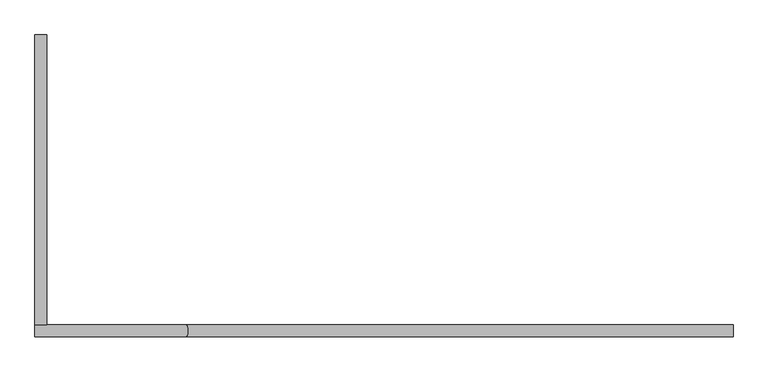
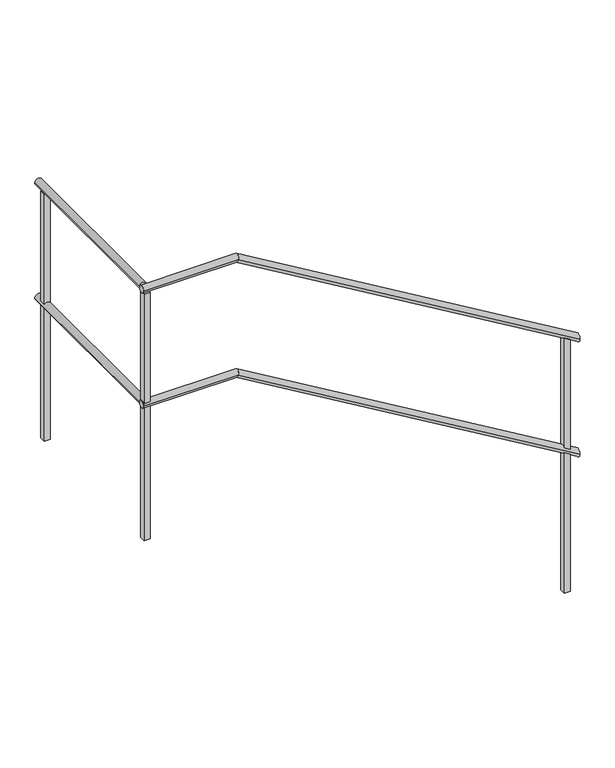
"""IFC4 building model written with IfcOpenShell, lengths in millimetres: railing geometry."""

from ifc_helpers import new_model, si_unit, frame, origin, place, context, project, spatial, polyline, circle_curve, ellipse_curve, outline, extrude, source, transform, mapped, element, save
from ifc_brep_helpers import plane_surface, cylinder_surface, advanced_brep


def railing_7296a36d(model_context):
    return source(origin(), model_context, "Body", "SolidModel", [
        advanced_brep(
        [(28067.5161135, 649.5208589, 1734.9618634), (28037.5161135, 649.5208589, 1734.9618634), (28067.5161135, -95.0791411, 1734.9618634), (28037.5161135, -95.0791411, 1734.9618634)],
        [
            (0, 1, circle_curve(frame((28052.5161135, 649.5208589, 1734.9618634), z_axis=(0.0, 1.0, 0.0), x_axis=(-1.0, 0.0, 0.0)), 15.0)),
            (1, 0, circle_curve(frame((28052.5161135, 649.5208589, 1734.9618634), z_axis=(0.0, 1.0, 0.0), x_axis=(-1.0, 0.0, 0.0)), 15.0)),
            (2, 3, circle_curve(frame((28052.5161135, -95.0791411, 1734.9618634), z_axis=(0.0, -1.0, 0.0), x_axis=(-1.0, 0.0, 0.0)), 15.0)),
            (3, 2, circle_curve(frame((28052.5161135, -95.0791411, 1734.9618634), z_axis=(0.0, -1.0, 0.0), x_axis=(-1.0, 0.0, 0.0)), 15.0)),
            (0, 2),
            (3, 1),
        ],
        [
            plane_surface(frame((28052.5161135, 649.5208589, 1749.9618634), z_axis=(0.0, 1.0, 0.0), x_axis=(0.0, 0.0, -1.0))),
            plane_surface(frame((28052.5161135, -95.0791411, 1749.9618634), z_axis=(0.0, -1.0, 0.0), x_axis=(0.0, 0.0, -1.0))),
            cylinder_surface(frame((28052.5161135, 649.5208589, 1734.9618634), z_axis=(0.0, 1.0, 0.0), x_axis=(-1.0, 0.0, 0.0)), 15.0),
        ],
        [
            (0, [[1, 2]]),
            (1, [[3, 4]]),
            (2, [[-1, 5, -4, 6]]),
            (2, [[-2, -6, -3, -5]]),
        ],
    ),
        advanced_brep(
        [(28037.5161135, -95.0791411, 1734.9618634), (28037.5161135, -125.0791411, 1734.9618634), (28425.8735614, -95.0791411, 1734.9618634), (28425.8735614, -125.0791411, 1734.9618634), (29830.0, -95.0791411, 899.1723166), (29830.0, -125.0791411, 899.1723166)],
        [
            (0, 1, circle_curve(frame((28037.5161135, -110.0791411, 1734.9618634), z_axis=(-1.0, 0.0, 0.0), x_axis=(0.0, -1.0, 0.0)), 15.0)),
            (1, 0, circle_curve(frame((28037.5161135, -110.0791411, 1734.9618634), z_axis=(-1.0, 0.0, 0.0), x_axis=(0.0, -1.0, 0.0)), 15.0)),
            (0, 2),
            (2, 3, ellipse_curve(frame((28425.8735614, -110.0791411, 1734.9618634), z_axis=(-0.9641817474962141, 0.0, 0.26524245096731175), x_axis=(-0.26524245096731197, 0.0, -0.964181747496214)), 15.5572329, 15.0)),
            (3, 1),
            (3, 2, ellipse_curve(frame((28425.8735614, -110.0791411, 1734.9618634), z_axis=(-0.9641817474962141, 0.0, 0.26524245096731175), x_axis=(-0.26524245096731197, 0.0, -0.964181747496214)), 15.5572329, 15.0)),
            (4, 5, ellipse_curve(frame((29830.0, -110.0791411, 899.1723166), z_axis=(1.0, 0.0, 0.0), x_axis=(0.0, 0.0, 1.0)), 17.4562134, 15.0)),
            (5, 4, ellipse_curve(frame((29830.0, -110.0791411, 899.1723166), z_axis=(1.0, 0.0, 0.0), x_axis=(0.0, 0.0, 1.0)), 17.4562134, 15.0)),
            (2, 4),
            (5, 3),
        ],
        [
            plane_surface(frame((28037.5161135, -110.0791411, 1749.9618634), z_axis=(-1.0, 0.0, 0.0), x_axis=(0.0, 1.0, 0.0))),
            cylinder_surface(frame((28037.5161135, -110.0791411, 1734.9618634), z_axis=(-1.0, 0.0, 0.0), x_axis=(0.0, -1.0, 0.0)), 15.0),
            plane_surface(frame((29830.0, -110.0791411, 916.62853), z_axis=(1.0, 0.0, 0.0), x_axis=(0.0, 1.0, 0.0))),
            cylinder_surface(frame((28422.3277421, -110.0791411, 1737.0724701), z_axis=(-0.8592928844097064, 0.0, 0.5114838597676831), x_axis=(0.0, -1.0, 0.0)), 15.0),
        ],
        [
            (0, [[1, 2]]),
            (1, [[-1, 3, 4, 5]]),
            (1, [[-2, -5, 6, -3]]),
            (2, [[7, 8]]),
            (3, [[-4, 9, -8, 10]]),
            (3, [[-6, -10, -7, -9]]),
        ],
    ),
        advanced_brep(
        [(28067.5161135, 649.5208589, 2234.9618634), (28037.5161135, 649.5208589, 2234.9618634), (28067.5161135, -95.0791411, 2234.9618634), (28037.5161135, -95.0791411, 2234.9618634)],
        [
            (0, 1, circle_curve(frame((28052.5161135, 649.5208589, 2234.9618634), z_axis=(0.0, 1.0, 0.0), x_axis=(-1.0, 0.0, 0.0)), 15.0)),
            (1, 0, circle_curve(frame((28052.5161135, 649.5208589, 2234.9618634), z_axis=(0.0, 1.0, 0.0), x_axis=(-1.0, 0.0, 0.0)), 15.0)),
            (2, 3, circle_curve(frame((28052.5161135, -95.0791411, 2234.9618634), z_axis=(0.0, -1.0, 0.0), x_axis=(-1.0, 0.0, 0.0)), 15.0)),
            (3, 2, circle_curve(frame((28052.5161135, -95.0791411, 2234.9618634), z_axis=(0.0, -1.0, 0.0), x_axis=(-1.0, 0.0, 0.0)), 15.0)),
            (0, 2),
            (3, 1),
        ],
        [
            plane_surface(frame((28052.5161135, 649.5208589, 2249.9618634), z_axis=(0.0, 1.0, 0.0), x_axis=(0.0, 0.0, -1.0))),
            plane_surface(frame((28052.5161135, -95.0791411, 2249.9618634), z_axis=(0.0, -1.0, 0.0), x_axis=(0.0, 0.0, -1.0))),
            cylinder_surface(frame((28052.5161135, 649.5208589, 2234.9618634), z_axis=(0.0, 1.0, 0.0), x_axis=(-1.0, 0.0, 0.0)), 15.0),
        ],
        [
            (0, [[1, 2]]),
            (1, [[3, 4]]),
            (2, [[-1, 5, -4, 6]]),
            (2, [[-2, -6, -3, -5]]),
        ],
    ),
        advanced_brep(
        [(28037.5161135, -95.0791411, 2234.9618634), (28037.5161135, -125.0791411, 2234.9618634), (28425.8735614, -95.0791411, 2234.9618634), (28425.8735614, -125.0791411, 2234.9618634), (29830.0, -95.0791411, 1399.1723166), (29830.0, -125.0791411, 1399.1723166)],
        [
            (0, 1, circle_curve(frame((28037.5161135, -110.0791411, 2234.9618634), z_axis=(-1.0, 0.0, 0.0), x_axis=(0.0, -1.0, 0.0)), 15.0)),
            (1, 0, circle_curve(frame((28037.5161135, -110.0791411, 2234.9618634), z_axis=(-1.0, 0.0, 0.0), x_axis=(0.0, -1.0, 0.0)), 15.0)),
            (0, 2),
            (2, 3, ellipse_curve(frame((28425.8735614, -110.0791411, 2234.9618634), z_axis=(-0.9641817474962141, 0.0, 0.26524245096731175), x_axis=(-0.26524245096731197, 0.0, -0.964181747496214)), 15.5572329, 15.0)),
            (3, 1),
            (3, 2, ellipse_curve(frame((28425.8735614, -110.0791411, 2234.9618634), z_axis=(-0.9641817474962141, 0.0, 0.26524245096731175), x_axis=(-0.26524245096731197, 0.0, -0.964181747496214)), 15.5572329, 15.0)),
            (4, 5, ellipse_curve(frame((29830.0, -110.0791411, 1399.1723166), z_axis=(1.0, 0.0, 0.0), x_axis=(0.0, 0.0, 1.0)), 17.4562134, 15.0)),
            (5, 4, ellipse_curve(frame((29830.0, -110.0791411, 1399.1723166), z_axis=(1.0, 0.0, 0.0), x_axis=(0.0, 0.0, 1.0)), 17.4562134, 15.0)),
            (2, 4),
            (5, 3),
        ],
        [
            plane_surface(frame((28037.5161135, -110.0791411, 2249.9618634), z_axis=(-1.0, 0.0, 0.0), x_axis=(0.0, 1.0, 0.0))),
            cylinder_surface(frame((28037.5161135, -110.0791411, 2234.9618634), z_axis=(-1.0, 0.0, 0.0), x_axis=(0.0, -1.0, 0.0)), 15.0),
            plane_surface(frame((29830.0, -110.0791411, 1416.62853), z_axis=(1.0, 0.0, 0.0), x_axis=(0.0, 1.0, 0.0))),
            cylinder_surface(frame((28422.3277421, -110.0791411, 2237.0724701), z_axis=(-0.8592928844097064, 0.0, 0.5114838597676831), x_axis=(0.0, -1.0, 0.0)), 15.0),
        ],
        [
            (0, [[1, 2]]),
            (1, [[-1, 3, 4, 5]]),
            (1, [[-2, -5, 6, -3]]),
            (2, [[7, 8]]),
            (3, [[-4, 9, -8, 10]]),
            (3, [[-6, -10, -7, -9]]),
        ],
    ),
        extrude(outline(polyline([(28040.0161135, -97.5791411), (28065.0161135, -97.5791411), (28065.0161135, -122.5791411), (28040.0161135, -122.5791411), (28040.0161135, -97.5791411)])), frame((0.0, 0.0, 1149.9618634), z_axis=(0.0, 0.0, 1.0), x_axis=(1.0, 0.0, 0.0)), (0.0, 0.0, 1.0), 1070.0),
        extrude(outline(polyline([(1423.830911, 29767.5), (316.62853, 29767.5), (316.62853, 29792.5), (1408.9499586, 29792.5), (1423.830911, 29767.5)])), frame((0.0, -122.5791411, 0.0), z_axis=(0.0, 1.0, 0.0), x_axis=(0.0, 0.0, 1.0)), (0.0, 0.0, 1.0), 25.0),
        extrude(outline(polyline([(28040.0161135, 612.0208589), (28065.0161135, 612.0208589), (28065.0161135, 587.0208589), (28040.0161135, 587.0208589), (28040.0161135, 612.0208589)])), frame((0.0, 0.0, 1149.9618634), z_axis=(0.0, 0.0, 1.0), x_axis=(1.0, 0.0, 0.0)), (0.0, 0.0, 1.0), 1070.0),
    ])


if __name__ == "__main__":
    model = new_model("IFC4")
    model_context = context("Model", 3, world=origin())
    ifc_project = project(units=[si_unit("LENGTHUNIT", "METRE", prefix="MILLI")], contexts=[model_context])
    site = spatial("IfcSite", under=ifc_project)
    building = spatial("IfcBuilding", under=site)
    placement = place(None, origin())
    railing_shape = railing_7296a36d(model_context)
    element("IfcRailing", 1, at=placement, inside=building, context=model_context, shape_type="MappedRepresentation", body=[
        mapped(railing_shape, transform((0.0, 0.0, 0.0), x_axis=(1.0, 0.0, 0.0), y_axis=(0.0, 1.0, 0.0), z_axis=(0.0, 0.0, 1.0))),
    ])
    save(model, "model.ifc")
